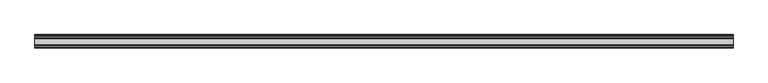
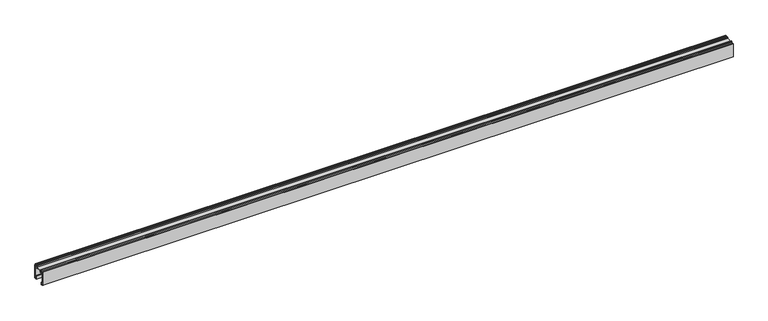
"""IFC4 building model written with IfcOpenShell, lengths in millimetres: proxy geometry, Generic Models 6:Generic Models 2:318829:Generic Models 2:318829 : Generic Models 6:Generic Models 2:318829:3 : Generic Models 6:Generic Models 2:318829:Generic Models 2:318829 : Generic Models 6:Generic Models 2:318829:300683."""

from ifc_helpers import new_model, si_unit, frame, origin, place, context, project, spatial, polyline, outline, extrude, source, transform, mapped, element, save


def generic_models_da89ecc2(model_context):
    return source(origin(), model_context, "Body", "SweptSolid", [
        extrude(outline(polyline([(-568243.8864799, 8558.1092863), (-568244.7459593, 8557.6326582), (-568244.7459593, 8556.5818712), (-568234.8444653, 8555.1673721), (-568234.8444653, 8553.7952232), (-568246.9989938, 8553.7952232), (-568246.9989938, 8509.2681457), (-568244.6866689, 8509.2681457), (-568244.6866689, 8504.9992381), (-568246.4653804, 8500.1374268), (-568244.6866689, 8499.8409748), (-568244.6866689, 8496.6985845), (-568250.1413841, 8496.6985845), (-568250.1413841, 8561.2065211), (-568246.9989938, 8561.2065211), (-568246.9989938, 8558.8941961), (-568245.5911171, 8558.8941961), (-568244.5777904, 8559.5528585), (-568243.8372354, 8559.0591552), (-568243.8864799, 8558.1092863)])), frame((592501.2930931, 0.0, 0.0), z_axis=(1.0, 0.0, 0.0), x_axis=(0.0, 1.0, 0.0)), (0.0, 0.0, 1.0), 3286.1430714),
        extrude(outline(polyline([(-568248.5289454, 8495.4622517), (-568248.5289454, 8496.5008648), (-568244.3960833, 8496.5008648), (-568244.3960833, 8500.2671026), (-568245.9381201, 8500.5241088), (-568244.3960833, 8504.7390095), (-568244.3960833, 8509.2681457), (-568243.1907793, 8509.2681457), (-568237.0974999, 8504.0194792), (-568237.0974999, 8492.4138662), (-568248.5289454, 8495.4622517)])), frame((592501.2930931, 0.0, 0.0), z_axis=(1.0, 0.0, 0.0), x_axis=(0.0, 1.0, 0.0)), (0.0, 0.0, 1.0), 3286.1430714),
        extrude(outline(polyline([(-568189.1908706, 8508.5566611), (-568189.1908706, 8551.4828983), (-568205.2585643, 8551.4828983), (-568205.2585643, 8558.3605827), (-568231.1684616, 8558.3605827), (-568231.1684616, 8551.4828983), (-568246.6432515, 8551.4828983), (-568246.6432515, 8553.0244482), (-568233.1843346, 8553.0244482), (-568233.1843346, 8558.3605827), (-568236.9196287, 8558.3605827), (-568238.2240171, 8559.6649711), (-568245.0424112, 8559.6649711), (-568245.9910573, 8559.0127769), (-568246.8211227, 8559.5463903), (-568246.8211227, 8560.9100691), (-568238.2240171, 8560.9100691), (-568238.2240171, 8567.1948497), (-568236.2081441, 8567.1948497), (-568236.2081441, 8560.9100691), (-568205.1399835, 8560.9100691), (-568205.1399835, 8567.1948497), (-568203.1241105, 8567.1948497), (-568203.1241105, 8560.9100691), (-568192.2146801, 8560.9100691), (-568192.2146801, 8567.1948497), (-568190.1988071, 8567.1948497), (-568190.1988071, 8560.9100691), (-568186.6413841, 8560.9100691), (-568186.6413841, 8498.4828372), (-568193.75623, 8497.8843922), (-568193.75623, 8502.9240747), (-568192.4518416, 8503.1467752), (-568192.4518416, 8501.1135517), (-568190.8611834, 8501.1135517), (-568189.9757617, 8503.0123447), (-568189.9757617, 8505.2937638), (-568190.969582, 8507.0151112), (-568192.4518416, 8507.0151112), (-568192.4518416, 8505.206794), (-568193.75623, 8506.5110665), (-568193.75623, 8508.5566611), (-568189.1908706, 8508.5566611)]), holes=[polyline([(-568189.7837744, 8558.7756154), (-568203.1241105, 8558.7756154), (-568203.1241105, 8553.0244482), (-568189.7837744, 8553.0244482), (-568189.7837744, 8558.7756154)])]), frame((592501.2930931, 0.0, 0.0), z_axis=(1.0, 0.0, 0.0), x_axis=(0.0, 1.0, 0.0)), (0.0, 0.0, 1.0), 3286.1430714),
        extrude(outline(polyline([(-568197.0974999, 8493.9040422), (-568197.0974999, 8508.5566611), (-568194.0630755, 8508.5566611), (-568194.0630755, 8506.3284212), (-568192.2246641, 8504.4900098), (-568192.2246641, 8506.744398), (-568191.1354772, 8506.744398), (-568190.2750289, 8505.2540577), (-568190.2750289, 8503.1737592), (-568191.1150744, 8501.3722756), (-568192.1394234, 8501.3722756), (-568192.1394234, 8503.410539), (-568194.0630755, 8503.0821106), (-568194.0630755, 8497.6418108), (-568187.1388605, 8498.2242214), (-568187.1388605, 8496.1228065), (-568197.0974999, 8493.9040422)])), frame((592501.2930931, 0.0, 0.0), z_axis=(1.0, 0.0, 0.0), x_axis=(0.0, 1.0, 0.0)), (0.0, 0.0, 1.0), 3286.1430714),
    ])


if __name__ == "__main__":
    model = new_model("IFC4")
    model_context = context("Model", 3, world=origin())
    ifc_project = project(units=[si_unit("LENGTHUNIT", "METRE", prefix="MILLI")], contexts=[model_context])
    site = spatial("IfcSite", under=ifc_project)
    building = spatial("IfcBuilding", under=site)
    placement = place(None, origin())
    generic_models_shape = generic_models_da89ecc2(model_context)
    element("IfcBuildingElementProxy", 1, Name="Generic Models 6:Generic Models 2:318829:Generic Models 2:318829 : Generic Models 6:Generic Models 2:318829:3 : Generic Models 6:Generic Models 2:318829:Generic Models 2:318829 : Generic Models 6:Generic Models 2:318829:300683", ObjectType="Generic Models 6:Generic Models 2:318829:Generic Models 2:318829 : Generic Models 6:Generic Models 2:318829:3 : Generic Models 6:Generic Models 2:318829:Generic Models 2:318829 : Generic Models 6:Generic Models 2:318829:300683", at=placement, inside=building, context=model_context, shape_type="MappedRepresentation", body=[
        mapped(generic_models_shape, transform((0.0, 0.0, 0.0), x_axis=(1.0, 0.0, 0.0), y_axis=(0.0, 1.0, 0.0), z_axis=(0.0, 0.0, 1.0))),
    ])
    save(model, "model.ifc")

# Revit data of these elements
# Type "Generic Models 6:Generic Models 2:318829:Generic Models 2:318829 : Generic Models 6:Generic Models 2:318829:3 : Generic Models 6:Generic Models 2:318829:Generic Models 2:318829 : Generic Models 6:Generic Models 2:318829:300683"
#   NameOverride = "Generic Models 6:Generic Models 2:318829:Generic Models 2:318829 : Generic Models 6:Generic Models 2:318829:300683"
#   ObjectTypeOverride = "Generic Models 2:318829 : Generic Models 6:Generic Models 2:318829"
#   Reference = "Generic Models 2"
#   Tag = "300683"
# Element 1 (IfcBuildingElementProxy, "Generic Models 6:Generic Models 2:318829:Generic Models 2:318829 : Generic Models 6:Generic Models 2:318829:3 : Generic Models 6:Generic Models 2:318829:Generic Models 2:318829 : Generic Models 6:Generic Models 2:318829:300683")
#   Materials on its faces: "THERMAL BROKEN ALUMINUM STOREFRONT FOR POLYCARBONATE"
# Materials
#   "THERMAL BROKEN ALUMINUM STOREFRONT FOR POLYCARBONATE": class "Unassigned", colour RGB 244 244 244, transparency 0, Keynote = "M07611300.01", Cost = 0
